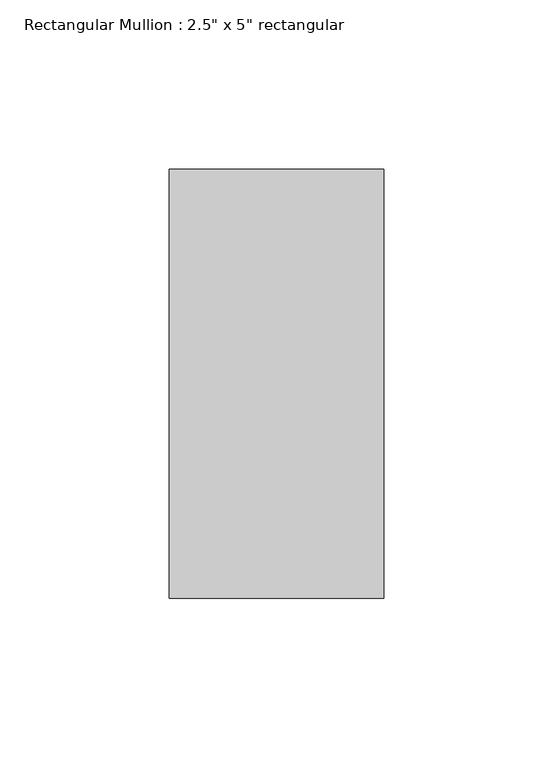
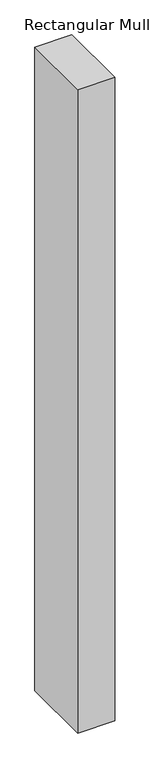
"""IFC4 building model written with IfcOpenShell, lengths in millimetres: member geometry."""

from ifc_helpers import new_model, si_unit, frame, origin, place, context, project, spatial, polyline, outline, extrude, source, transform, mapped, element, save


def member_f0de6b6c(model_context):
    return source(origin(), model_context, "Body", "SweptSolid", [
        extrude(outline(polyline([(0.0, 63.5), (0.0, -63.5), (-63.5, -63.5), (-63.5, 63.5), (0.0, 63.5)])), frame((0.0, 0.0, -1166.2833333), z_axis=(0.0, 0.0, 1.0), x_axis=(1.0, 0.0, 0.0)), (0.0, 0.0, 1.0), 1166.2833333),
    ])


if __name__ == "__main__":
    model = new_model("IFC4")
    model_context = context("Model", 3, world=origin())
    ifc_project = project(units=[si_unit("LENGTHUNIT", "METRE", prefix="MILLI")], contexts=[model_context])
    site = spatial("IfcSite", under=ifc_project)
    building = spatial("IfcBuilding", under=site)
    placement = place(None, origin())
    member_shape = member_f0de6b6c(model_context)
    element("IfcMember", 1, ObjectType="Rectangular Mullion : 2.5\" x 5\" rectangular", at=placement, inside=building, context=model_context, shape_type="MappedRepresentation", body=[
        mapped(member_shape, transform((0.0, 0.0, 0.0), x_axis=(1.0, 0.0, 0.0), y_axis=(0.0, 1.0, 0.0), z_axis=(0.0, 0.0, 1.0))),
    ])
    save(model, "model.ifc")

# Revit data of these elements
# Type "Rectangular Mullion : 2.5\" x 5\" rectangular"
#   built-in parameter 1007304 = 0.416667 (stored number, unit not read)
#   built-in parameter 1007301 = 0.104167 (stored number, unit not read)
#   built-in parameter 1007300 = 0.104167 (stored number, unit not read)
